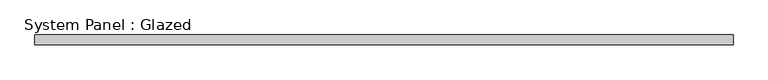
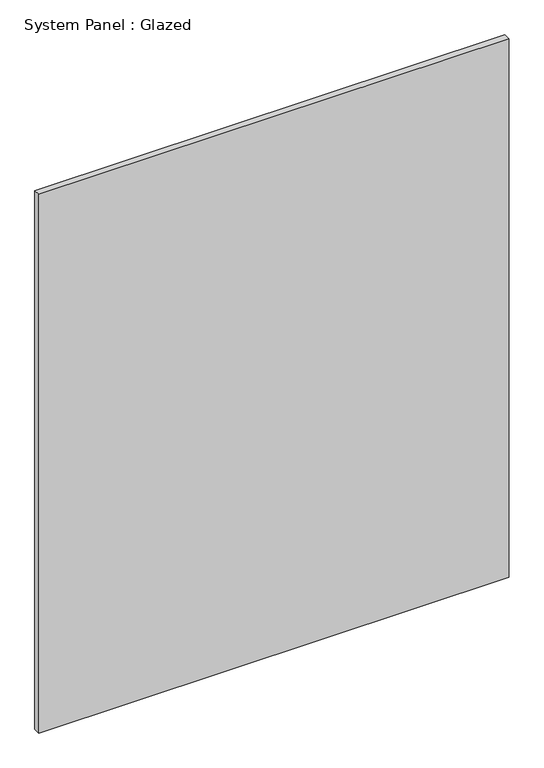
"""IFC4 building model written with IfcOpenShell, lengths in millimetres: plate geometry, System Panel : Glazed."""

import ifcopenshell
import ifcopenshell.guid

model = None  # the IFC model being written
_history = None  # IfcOwnerHistory: only IFC2X3 demands one
_inside = {}  # id of a spatial element -> (the spatial element, [elements in it])
_under = {}  # id of a project, library or spatial element -> (it, [spatial elements below it])
_declared = {}  # id of a project -> (the project, [libraries it declares])
_typed = {}  # id of a type object -> (the type object, [elements of that type])
_made_of = {}  # id of a material, layer set ... -> (it, [elements and type objects made of it])


def new_model(schema):
    """Start an empty IFC model of exactly this schema.

    Asked for "IFC4X3", IfcOpenShell would pick the latest addendum, in which some entities
    have other attributes; the version numbers below select the first issue.
    IFC2X3 requires an IfcOwnerHistory on every rooted entity: one is made here for all.
    """
    global model, _history
    if schema == "IFC4X3":
        model = ifcopenshell.file(schema_version=(4, 3, 0, 0))
    else:
        model = ifcopenshell.file(schema=schema)
    _inside.clear()
    _under.clear()
    _declared.clear()
    _typed.clear()
    _made_of.clear()
    _history = None
    if model.schema == "IFC2X3":
        org = make("IfcOrganization", Name="unknown")
        user = make(
            "IfcPersonAndOrganization",
            ThePerson=make("IfcPerson", FamilyName="unknown"),
            TheOrganization=org,
        )
        app = make(
            "IfcApplication",
            ApplicationDeveloper=org,
            Version="unknown",
            ApplicationFullName="unknown",
            ApplicationIdentifier="unknown",
        )
        _history = make(
            "IfcOwnerHistory",
            OwningUser=user,
            OwningApplication=app,
            ChangeAction="ADDED",
            CreationDate=0,
        )
    return model


def make(cls, **values):
    """One entity of the class cls with the attributes given. An attribute that is None is left unset."""
    return model.create_entity(
        cls, **{name: value for name, value in values.items() if value is not None}
    )


def rooted(cls, **values):
    """An entity with a GlobalId (a new one), such as an element, a storey or a relation."""
    return make(cls, GlobalId=ifcopenshell.guid.new(), OwnerHistory=_history, **values)


def si_unit(unit_type, name, prefix=None):
    """IfcSIUnit, for example si_unit("LENGTHUNIT", "METRE", prefix="MILLI")."""
    return make("IfcSIUnit", UnitType=unit_type, Prefix=prefix, Name=name)


def assignment(units):
    """IfcUnitAssignment: the units of a project."""
    return None if units is None else make("IfcUnitAssignment", Units=units)


def point(xyz):
    """IfcCartesianPoint."""
    return None if xyz is None else make("IfcCartesianPoint", Coordinates=xyz)


def direction(xyz):
    """IfcDirection."""
    return None if xyz is None else make("IfcDirection", DirectionRatios=xyz)


def frame(location, z_axis=None, x_axis=None):
    """IfcAxis2Placement3D, a coordinate frame: its origin and axes. An axis left out is left unset."""
    return make(
        "IfcAxis2Placement3D",
        Location=point(location),
        Axis=direction(z_axis),
        RefDirection=direction(x_axis),
    )


def origin():
    """The frame at (0, 0, 0) with its axes left unset."""
    return frame((0.0, 0.0, 0.0))


def origin_with_axes():
    """The frame at (0, 0, 0) with the z axis (0, 0, 1) and the x axis (1, 0, 0) written out."""
    return frame((0.0, 0.0, 0.0), z_axis=(0.0, 0.0, 1.0), x_axis=(1.0, 0.0, 0.0))


def place(relative_to, where):
    """IfcLocalPlacement: puts the frame where relative to a parent placement (None: the world)."""
    return make(
        "IfcLocalPlacement", PlacementRelTo=relative_to, RelativePlacement=where
    )


def context(
    kind, dimensions, precision=None, world=None, true_north=None, identifier=None
):
    """IfcGeometricRepresentationContext, for example the 3D "Model" context."""
    return make(
        "IfcGeometricRepresentationContext",
        ContextIdentifier=identifier,
        ContextType=kind,
        CoordinateSpaceDimension=dimensions,
        Precision=precision,
        WorldCoordinateSystem=world,
        TrueNorth=true_north,
    )


def project(units=None, contexts=None):
    """IfcProject with its units and contexts."""
    return rooted(
        "IfcProject",
        Name="project",
        RepresentationContexts=contexts,
        UnitsInContext=assignment(units),
    )


def spatial(cls, under=None, at=None, **own):
    """A site, building, storey or space (cls), placed at a placement, below another one or the project."""
    s = rooted(cls, ObjectPlacement=at, **own)
    if under is not None:
        _under.setdefault(under.id(), (under, []))[1].append(s)
    return s


def polyline(points):
    """IfcPolyline through the points."""
    return make("IfcPolyline", Points=[point(p) for p in points])


def outline(outer, holes=None, kind="AREA"):
    """IfcArbitraryClosedProfileDef: a profile drawn as a closed curve; with holes, ...WithVoids."""
    if holes is None:
        return make("IfcArbitraryClosedProfileDef", ProfileType=kind, OuterCurve=outer)
    return make(
        "IfcArbitraryProfileDefWithVoids",
        ProfileType=kind,
        OuterCurve=outer,
        InnerCurves=holes,
    )


def extrude(swept, where, along, depth):
    """IfcExtrudedAreaSolid: the profile swept, set in the frame where, extruded along a direction by depth."""
    return make(
        "IfcExtrudedAreaSolid",
        SweptArea=swept,
        Position=where,
        ExtrudedDirection=direction(along),
        Depth=depth,
    )


def shape(context_of_items, identifier, shape_type, items):
    """IfcShapeRepresentation: the items that make up one representation, for example the "Body"."""
    return make(
        "IfcShapeRepresentation",
        ContextOfItems=context_of_items,
        RepresentationIdentifier=identifier,
        RepresentationType=shape_type,
        Items=items,
    )


def source(mapping_origin, context_of_items, identifier, shape_type, items):
    """IfcRepresentationMap: a shape defined once, which mapped items show again and again."""
    return make(
        "IfcRepresentationMap",
        MappingOrigin=mapping_origin,
        MappedRepresentation=shape(context_of_items, identifier, shape_type, items),
    )


def transform(
    local_origin,
    x_axis=None,
    y_axis=None,
    z_axis=None,
    scale=None,
    scale2=None,
    scale3=None,
    uniform=True,
):
    """IfcCartesianTransformationOperator3D, or its non-uniform kind. x_axis, y_axis, z_axis: its Axis1, 2, 3."""
    if uniform:
        return make(
            "IfcCartesianTransformationOperator3D",
            Axis1=direction(x_axis),
            Axis2=direction(y_axis),
            LocalOrigin=point(local_origin),
            Scale=scale,
            Axis3=direction(z_axis),
        )
    return make(
        "IfcCartesianTransformationOperator3DnonUniform",
        Axis1=direction(x_axis),
        Axis2=direction(y_axis),
        LocalOrigin=point(local_origin),
        Scale=scale,
        Axis3=direction(z_axis),
        Scale2=scale2,
        Scale3=scale3,
    )


def mapped(mapping_source, mapping_target):
    """IfcMappedItem: shows the shape of a source again, moved by a transform."""
    return make(
        "IfcMappedItem", MappingSource=mapping_source, MappingTarget=mapping_target
    )


def made_of(thing, what):
    """Note that an element or type object is made of a material, layer set ...; save() writes the relation."""
    if what is not None:
        _made_of.setdefault(what.id(), (what, []))[1].append(thing)
    return thing


def element(
    cls,
    number,
    at=None,
    inside=None,
    cuts=None,
    type_object=None,
    material=None,
    context=None,
    identifier="Body",
    shape_type=None,
    held_by="IfcProductDefinitionShape",
    body=None,
    shapes=None,
    **own,
):
    """One element of the class cls, such as IfcWall. Its Tag is "e" and its number.

    at: its placement. inside: the storey or other place that contains it. cuts: it is an
    opening in that element (IfcRelVoidsElement). A single representation is given by context,
    identifier, shape_type and body (its items); several are given by shapes. held_by: the class
    of the entity that holds the representations. save() writes the other relations.
    """
    e = rooted(cls, Tag="e%d" % number, ObjectPlacement=at, **own)
    if body is not None:
        shapes = [shape(context, identifier, shape_type, body)]
    if shapes is not None:
        e.Representation = make(held_by, Representations=shapes)
    if inside is not None:
        _inside.setdefault(inside.id(), (inside, []))[1].append(e)
    if cuts is not None:
        rooted(
            "IfcRelVoidsElement", RelatingBuildingElement=cuts, RelatedOpeningElement=e
        )
    if type_object is not None:
        _typed.setdefault(type_object.id(), (type_object, []))[1].append(e)
    return made_of(e, material)


def aggregate(whole, parts):
    """IfcRelAggregates: a whole, such as a stair, and the parts it consists of."""
    return rooted("IfcRelAggregates", RelatingObject=whole, RelatedObjects=parts)


def save(model, path):
    """Write the relations noted so far, then the file.

    IfcRelAggregates (storeys below a building ...), IfcRelContainedInSpatialStructure (elements
    in a storey), IfcRelDefinesByType, IfcRelAssociatesMaterial and IfcRelDeclares: one each for
    every whole, place, type object, material and project.
    """
    for whole, parts in _under.values():
        aggregate(whole, parts)
    for where, things in _inside.values():
        rooted(
            "IfcRelContainedInSpatialStructure",
            RelatedElements=things,
            RelatingStructure=where,
        )
    for kind, things in _typed.values():
        rooted("IfcRelDefinesByType", RelatedObjects=things, RelatingType=kind)
    for what, things in _made_of.values():
        rooted("IfcRelAssociatesMaterial", RelatedObjects=things, RelatingMaterial=what)
    for by, libraries in _declared.values():
        rooted("IfcRelDeclares", RelatingContext=by, RelatedDefinitions=libraries)
    model.write(path)


def system_panel_glazed_53184239(model_context):
    return source(origin(), model_context, "Body", "SweptSolid", [
        extrude(outline(polyline([(887.9485033, -49.5), (-887.9485033, -49.5), (-887.9485033, -24.5), (887.9485033, -24.5), (887.9485033, -49.5)])), origin_with_axes(), (0.0, 0.0, 1.0), 2150.0),
    ])


if __name__ == "__main__":
    model = new_model("IFC4")
    model_context = context("Model", 3, world=origin())
    ifc_project = project(units=[si_unit("LENGTHUNIT", "METRE", prefix="MILLI")], contexts=[model_context])
    site = spatial("IfcSite", under=ifc_project)
    building = spatial("IfcBuilding", under=site)
    placement = place(None, origin())
    system_panel_glazed_shape = system_panel_glazed_53184239(model_context)
    element("IfcPlate", 1, ObjectType="System Panel : Glazed", at=placement, inside=building, context=model_context, shape_type="MappedRepresentation", body=[
        mapped(system_panel_glazed_shape, transform((0.0, 0.0, 0.0), x_axis=(1.0, 0.0, 0.0), y_axis=(0.0, 1.0, 0.0), z_axis=(0.0, 0.0, 1.0))),
    ])
    save(model, "model.ifc")

# Revit data of these elements
# Type "System Panel : Glazed"
#   Keynote = "H11"
#   Construction Type Id = "GSP4R"
#   Analytic Construction = "1/8 in Pilkington single glazing"
#   Visual Light Transmittance = 0.9
#   Solar Heat Gain Coefficient = 0.86
#   Heat Transfer Coefficient (U) = 6.7069 W/(m²·K)
# Element 1 (IfcPlate, "System Panel : Glazed")
#   Materials on its faces: "Glass"
# Materials
#   "Glass": class "Glass", colour RGB 0 128 192, transparency 0.9, Description = "Soda Lime Glass", Cost = 0
